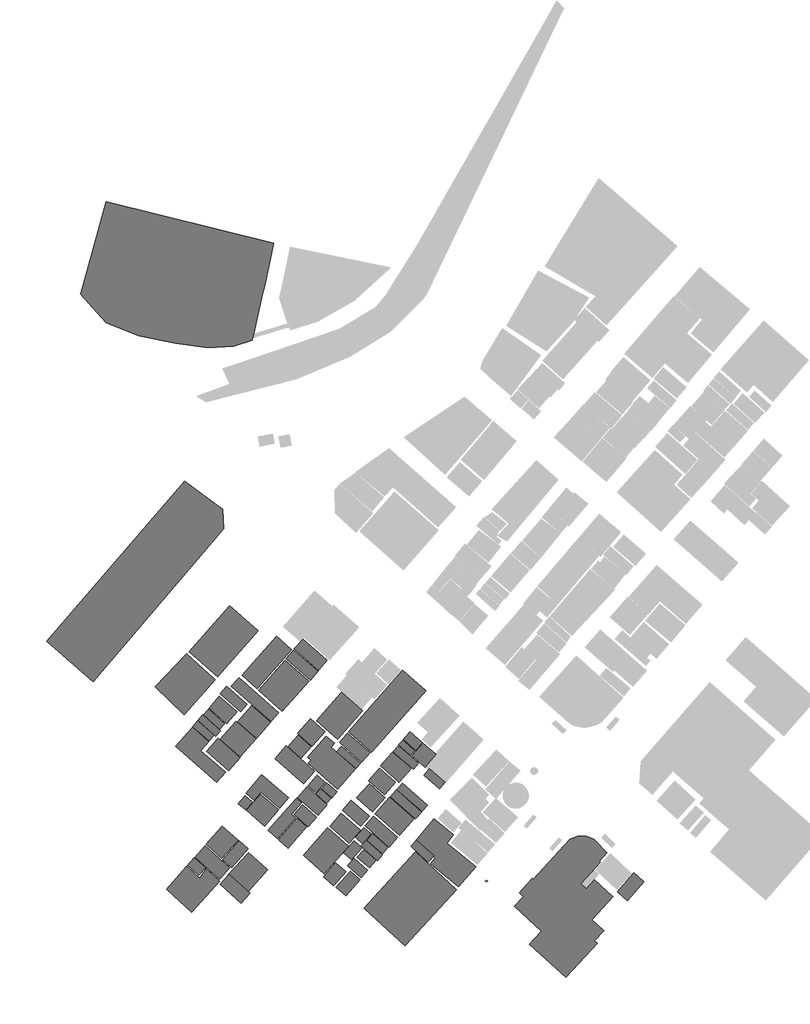
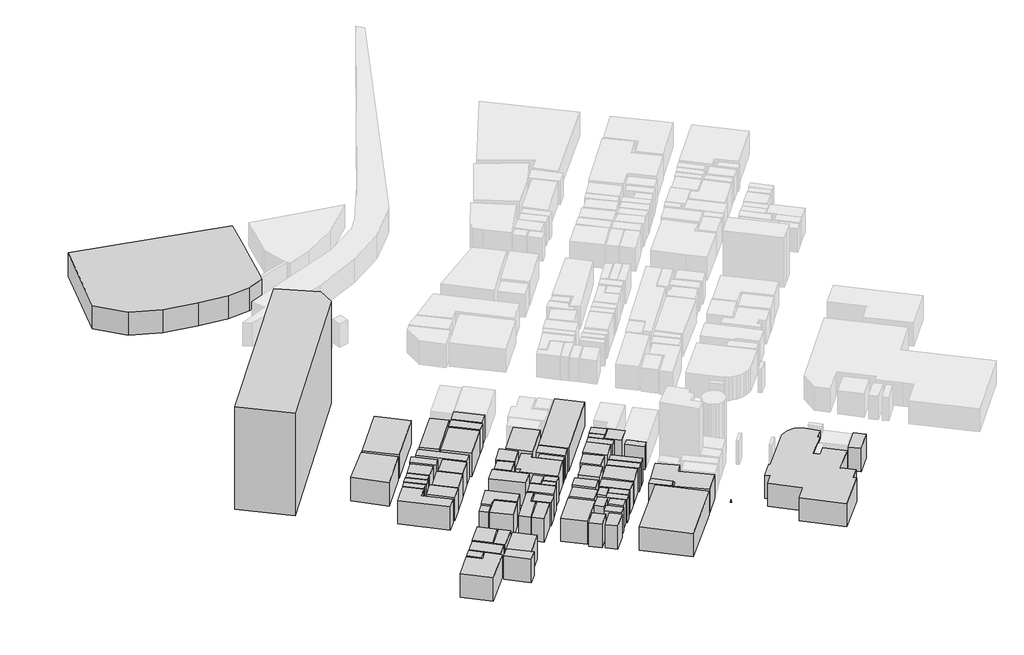
# One storey, part 1 of 3: 72 proxies.
"""IFC4 building model written with IfcOpenShell, lengths in millimetres."""

import ifcopenshell
import ifcopenshell.guid

model = None  # the IFC model being written
_history = None  # IfcOwnerHistory: only IFC2X3 demands one
_inside = {}  # id of a spatial element -> (the spatial element, [elements in it])
_under = {}  # id of a project, library or spatial element -> (it, [spatial elements below it])
_declared = {}  # id of a project -> (the project, [libraries it declares])
_typed = {}  # id of a type object -> (the type object, [elements of that type])
_made_of = {}  # id of a material, layer set ... -> (it, [elements and type objects made of it])


def new_model(schema):
    """Start an empty IFC model of exactly this schema.

    Asked for "IFC4X3", IfcOpenShell would pick the latest addendum, in which some entities
    have other attributes; the version numbers below select the first issue.
    IFC2X3 requires an IfcOwnerHistory on every rooted entity: one is made here for all.
    """
    global model, _history
    if schema == "IFC4X3":
        model = ifcopenshell.file(schema_version=(4, 3, 0, 0))
    else:
        model = ifcopenshell.file(schema=schema)
    _inside.clear()
    _under.clear()
    _declared.clear()
    _typed.clear()
    _made_of.clear()
    _history = None
    if model.schema == "IFC2X3":
        org = make("IfcOrganization", Name="unknown")
        user = make(
            "IfcPersonAndOrganization",
            ThePerson=make("IfcPerson", FamilyName="unknown"),
            TheOrganization=org,
        )
        app = make(
            "IfcApplication",
            ApplicationDeveloper=org,
            Version="unknown",
            ApplicationFullName="unknown",
            ApplicationIdentifier="unknown",
        )
        _history = make(
            "IfcOwnerHistory",
            OwningUser=user,
            OwningApplication=app,
            ChangeAction="ADDED",
            CreationDate=0,
        )
    return model


def make(cls, **values):
    """One entity of the class cls with the attributes given. An attribute that is None is left unset."""
    return model.create_entity(
        cls, **{name: value for name, value in values.items() if value is not None}
    )


def rooted(cls, **values):
    """An entity with a GlobalId (a new one), such as an element, a storey or a relation."""
    return make(cls, GlobalId=ifcopenshell.guid.new(), OwnerHistory=_history, **values)


def si_unit(unit_type, name, prefix=None):
    """IfcSIUnit, for example si_unit("LENGTHUNIT", "METRE", prefix="MILLI")."""
    return make("IfcSIUnit", UnitType=unit_type, Prefix=prefix, Name=name)


def assignment(units):
    """IfcUnitAssignment: the units of a project."""
    return None if units is None else make("IfcUnitAssignment", Units=units)


def point(xyz):
    """IfcCartesianPoint."""
    return None if xyz is None else make("IfcCartesianPoint", Coordinates=xyz)


def direction(xyz):
    """IfcDirection."""
    return None if xyz is None else make("IfcDirection", DirectionRatios=xyz)


def frame(location, z_axis=None, x_axis=None):
    """IfcAxis2Placement3D, a coordinate frame: its origin and axes. An axis left out is left unset."""
    return make(
        "IfcAxis2Placement3D",
        Location=point(location),
        Axis=direction(z_axis),
        RefDirection=direction(x_axis),
    )


def origin():
    """The frame at (0, 0, 0) with its axes left unset."""
    return frame((0.0, 0.0, 0.0))


def origin_with_axes():
    """The frame at (0, 0, 0) with the z axis (0, 0, 1) and the x axis (1, 0, 0) written out."""
    return frame((0.0, 0.0, 0.0), z_axis=(0.0, 0.0, 1.0), x_axis=(1.0, 0.0, 0.0))


def place(relative_to, where):
    """IfcLocalPlacement: puts the frame where relative to a parent placement (None: the world)."""
    return make(
        "IfcLocalPlacement", PlacementRelTo=relative_to, RelativePlacement=where
    )


def context(
    kind, dimensions, precision=None, world=None, true_north=None, identifier=None
):
    """IfcGeometricRepresentationContext, for example the 3D "Model" context."""
    return make(
        "IfcGeometricRepresentationContext",
        ContextIdentifier=identifier,
        ContextType=kind,
        CoordinateSpaceDimension=dimensions,
        Precision=precision,
        WorldCoordinateSystem=world,
        TrueNorth=true_north,
    )


def project(units=None, contexts=None):
    """IfcProject with its units and contexts."""
    return rooted(
        "IfcProject",
        Name="project",
        RepresentationContexts=contexts,
        UnitsInContext=assignment(units),
    )


def spatial(cls, under=None, at=None, **own):
    """A site, building, storey or space (cls), placed at a placement, below another one or the project."""
    s = rooted(cls, ObjectPlacement=at, **own)
    if under is not None:
        _under.setdefault(under.id(), (under, []))[1].append(s)
    return s


def polyline(points):
    """IfcPolyline through the points."""
    return make("IfcPolyline", Points=[point(p) for p in points])


def point_list(points):
    """IfcCartesianPointList2D or 3D."""
    cls = (
        "IfcCartesianPointList2D" if len(points[0]) == 2 else "IfcCartesianPointList3D"
    )
    return make(cls, CoordList=points)


def outline(outer, holes=None, kind="AREA"):
    """IfcArbitraryClosedProfileDef: a profile drawn as a closed curve; with holes, ...WithVoids."""
    if holes is None:
        return make("IfcArbitraryClosedProfileDef", ProfileType=kind, OuterCurve=outer)
    return make(
        "IfcArbitraryProfileDefWithVoids",
        ProfileType=kind,
        OuterCurve=outer,
        InnerCurves=holes,
    )


def extrude(swept, where, along, depth):
    """IfcExtrudedAreaSolid: the profile swept, set in the frame where, extruded along a direction by depth."""
    return make(
        "IfcExtrudedAreaSolid",
        SweptArea=swept,
        Position=where,
        ExtrudedDirection=direction(along),
        Depth=depth,
    )


def triangles(points, corners, closed=None, point_numbers=None):
    """IfcTriangulatedFaceSet: each triangle names its three corners, points numbered from 1."""
    return make(
        "IfcTriangulatedFaceSet",
        Coordinates=point_list(points),
        Closed=closed,
        CoordIndex=corners,
        PnIndex=point_numbers,
    )


def shape(context_of_items, identifier, shape_type, items):
    """IfcShapeRepresentation: the items that make up one representation, for example the "Body"."""
    return make(
        "IfcShapeRepresentation",
        ContextOfItems=context_of_items,
        RepresentationIdentifier=identifier,
        RepresentationType=shape_type,
        Items=items,
    )


def source(mapping_origin, context_of_items, identifier, shape_type, items):
    """IfcRepresentationMap: a shape defined once, which mapped items show again and again."""
    return make(
        "IfcRepresentationMap",
        MappingOrigin=mapping_origin,
        MappedRepresentation=shape(context_of_items, identifier, shape_type, items),
    )


def transform(
    local_origin,
    x_axis=None,
    y_axis=None,
    z_axis=None,
    scale=None,
    scale2=None,
    scale3=None,
    uniform=True,
):
    """IfcCartesianTransformationOperator3D, or its non-uniform kind. x_axis, y_axis, z_axis: its Axis1, 2, 3."""
    if uniform:
        return make(
            "IfcCartesianTransformationOperator3D",
            Axis1=direction(x_axis),
            Axis2=direction(y_axis),
            LocalOrigin=point(local_origin),
            Scale=scale,
            Axis3=direction(z_axis),
        )
    return make(
        "IfcCartesianTransformationOperator3DnonUniform",
        Axis1=direction(x_axis),
        Axis2=direction(y_axis),
        LocalOrigin=point(local_origin),
        Scale=scale,
        Axis3=direction(z_axis),
        Scale2=scale2,
        Scale3=scale3,
    )


def mapped(mapping_source, mapping_target):
    """IfcMappedItem: shows the shape of a source again, moved by a transform."""
    return make(
        "IfcMappedItem", MappingSource=mapping_source, MappingTarget=mapping_target
    )


def made_of(thing, what):
    """Note that an element or type object is made of a material, layer set ...; save() writes the relation."""
    if what is not None:
        _made_of.setdefault(what.id(), (what, []))[1].append(thing)
    return thing


def element(
    cls,
    number,
    at=None,
    inside=None,
    cuts=None,
    type_object=None,
    material=None,
    context=None,
    identifier="Body",
    shape_type=None,
    held_by="IfcProductDefinitionShape",
    body=None,
    shapes=None,
    **own,
):
    """One element of the class cls, such as IfcWall. Its Tag is "e" and its number.

    at: its placement. inside: the storey or other place that contains it. cuts: it is an
    opening in that element (IfcRelVoidsElement). A single representation is given by context,
    identifier, shape_type and body (its items); several are given by shapes. held_by: the class
    of the entity that holds the representations. save() writes the other relations.
    """
    e = rooted(cls, Tag="e%d" % number, ObjectPlacement=at, **own)
    if body is not None:
        shapes = [shape(context, identifier, shape_type, body)]
    if shapes is not None:
        e.Representation = make(held_by, Representations=shapes)
    if inside is not None:
        _inside.setdefault(inside.id(), (inside, []))[1].append(e)
    if cuts is not None:
        rooted(
            "IfcRelVoidsElement", RelatingBuildingElement=cuts, RelatedOpeningElement=e
        )
    if type_object is not None:
        _typed.setdefault(type_object.id(), (type_object, []))[1].append(e)
    return made_of(e, material)


def aggregate(whole, parts):
    """IfcRelAggregates: a whole, such as a stair, and the parts it consists of."""
    return rooted("IfcRelAggregates", RelatingObject=whole, RelatedObjects=parts)


def save(model, path):
    """Write the relations noted so far, then the file.

    IfcRelAggregates (storeys below a building ...), IfcRelContainedInSpatialStructure (elements
    in a storey), IfcRelDefinesByType, IfcRelAssociatesMaterial and IfcRelDeclares: one each for
    every whole, place, type object, material and project.
    """
    for whole, parts in _under.values():
        aggregate(whole, parts)
    for where, things in _inside.values():
        rooted(
            "IfcRelContainedInSpatialStructure",
            RelatedElements=things,
            RelatingStructure=where,
        )
    for kind, things in _typed.values():
        rooted("IfcRelDefinesByType", RelatedObjects=things, RelatingType=kind)
    for what, things in _made_of.values():
        rooted("IfcRelAssociatesMaterial", RelatedObjects=things, RelatingMaterial=what)
    for by, libraries in _declared.values():
        rooted("IfcRelDeclares", RelatingContext=by, RelatedDefinitions=libraries)
    model.write(path)


def m_rpc_female_e5f04239(model_context):
    return source(origin(), model_context, "Body", "Tessellation", [
        triangles([(-437.3057565, 0.0, 2.93e-05), (-425.7448342, -100.2015691, 2.93e-05), (-392.8194094, -192.2206799, 2.93e-05), (-341.1658762, -273.4208834, 2.93e-05), (-273.4209015, -341.1659489, 2.93e-05), (-192.2206254, -392.819373, 2.93e-05), (-100.2015237, -425.7447979, 2.93e-05), (1.91e-05, -437.3057565, 2.93e-05), (100.2015782, -425.7448342, 2.93e-05), (192.220698, -392.8194094, 2.93e-05), (273.4209015, -341.1658762, 2.93e-05), (341.1660215, -273.4209015, 2.93e-05), (392.819373, -192.2206072, 2.93e-05), (425.7447979, -100.2014965, 2.93e-05), (437.3057565, 3.36e-05, 2.93e-05), (-5.73e-05, 437.3057928, 2.93e-05), (-5.5814555, 72.246871, 69.496344), (-5.5814561, 67.031142, 46.0256608), (-5.5814583, 124.4039254, 19.9471336), (-5.5814583, 129.6196318, 25.1628196), (-5.5814566, 107.6002273, 62.2269385), (-5.5814561, 95.7175496, 74.7120321), (-5.5814561, -28.6037069, 4.4e-06), (-5.5814555, -39.8908654, 35.5942482), (-5.5814555, -42.4985551, 37.2668205), (-5.5814544, -45.6385706, 39.1828009), (-5.5814544, -48.9915363, 41.1595652), (-5.5814544, -52.2381223, 43.0148345), (-5.5814544, -55.0589122, 44.56573), (-5.5814544, -57.1346076, 45.6302408), (-5.5814544, -58.1458059, 46.0256654), (-5.5814555, -58.1458876, 5.3e-06), (-5.5814555, -108.9534241, 6.8e-06), (-5.5814544, -116.5758149, 29.8220214), (-5.5814504, -109.3236867, 163.616957), (-5.5814413, -45.457159, 488.7457126), (-5.5814407, -47.714434, 510.223653), (-5.5814407, -52.9301222, 512.8314517), (-5.5814407, -176.6935208, 461.1352976), (-5.5814373, -431.0100652, 441.4516517), (-5.5814373, -446.7160832, 445.0273055), (-5.5814368, -456.1585665, 455.8251566), (-5.58143, -511.6809405, 636.0529638), (-5.581426, -514.5203021, 776.2247131), (-5.5814186, -566.7671494, 1012.4528812), (-5.5814158, -561.4616592, 1112.6378271), (-5.5814129, -522.3438071, 1198.6970364), (-5.5814129, -544.7658397, 1204.5966036), (-5.5814118, -561.2097487, 1214.9815075), (-5.5814118, -573.9143148, 1236.2570984), (-5.5814101, -577.4586843, 1272.8740494), (-5.5814084, -566.4219306, 1329.2825249), (-5.5814067, -535.3830912, 1409.9332706), (-5.5814067, -516.7872059, 1433.7636475), (-5.5814055, -472.5754423, 1474.3204742), (-5.5814055, -445.9832065, 1486.7813416), (-5.5814067, -415.7490417, 1491.1880493), (-5.5814067, -381.3846422, 1485.4068615), (-5.5814084, -308.1102631, 1450.1703495), (-5.5814101, -271.6907746, 1426.3735462), (-5.5814107, -259.9822778, 1410.5514015), (-5.5814118, -256.5008769, 1391.3528641), (-5.5814118, -264.1662884, 1368.2074745), (-5.5814118, -270.5525991, 1361.5164585), (-5.5814118, -307.4893707, 1345.9730759), (-5.5814118, -313.6895373, 1341.0963387), (-5.5814118, -316.3233519, 1334.3053288), (-5.5814129, -314.5104538, 1321.5896805), (-5.5814141, -303.2841405, 1289.971843), (-5.5814141, -303.9328654, 1281.3184467), (-5.5814146, -344.8551496, 1227.4567635), (-5.5814158, -350.2254976, 1216.9519541), (-5.5814158, -354.0100413, 1213.137216), (-5.5814158, -360.9104559, 1211.8311184), (-5.5814146, -397.1668911, 1216.9519541), (-5.5814158, -412.8139375, 1162.1870556), (-5.581422, -300.7217424, 1007.464959), (-5.581426, -262.9222146, 903.7019611), (-5.5814277, -261.5584715, 849.2446747), (-5.58143, -151.2454102, 828.1022152), (-5.58143, -131.1657765, 828.3817766), (-5.5814288, -146.9133073, 873.4847649), (-5.5814288, -146.8129046, 875.3230974), (-5.5814288, -136.5283852, 880.5989382), (-5.581426, 66.2908528, 1062.7618744), (-5.581426, 72.9541861, 1068.1172161), (-5.5814266, 85.3175848, 1063.7719145), (-5.5814322, 186.9119923, 916.7356859), (-5.5814328, 189.6002729, 904.0095005), (-5.5814339, 74.8547106, 802.3032812), (-5.5814345, 53.5231683, 768.5290346), (-5.5814345, 40.9526102, 757.9697954), (-5.5814345, 7.0502408, 750.1462177), (-5.5814362, -30.7395663, 681.3427139), (-5.5814362, -32.0672787, 677.1262562), (-5.5814368, -2.7970168, 673.1418337), (-5.5814379, 74.8547106, 666.6947708), (-5.5814566, 223.5023279, 113.8298615), (-5.5814572, 192.3027606, 86.4272282), (-5.5814572, 189.6002729, 82.5355962), (-5.5814595, 257.4045281, 53.849234), (-5.5814595, 261.0572667, 50.6335418), (-5.5814595, 266.9932234, 41.9573409), (-5.58146, 270.4022813, 33.1798288), (-5.58146, 270.8965462, 29.8373185), (-5.58146, 270.443685, 27.7706614), (-5.58146, 262.21192, 24.6723971), (-5.5814583, 148.3989361, 17.7234776), (-5.5814583, 129.6196318, 12.1235594), (-5.5814583, 119.2279423, 0.0), (-103.2161017, -158.8625416, 3.138314), (-93.5649194, -158.8625416, 19.242982), (-88.6211895, -158.8625416, 24.4594286), (-82.9717796, -158.8625416, 28.4095146), (-76.7113605, -158.8625416, 30.3784918), (-108.0056168, -158.8625779, 484.1449396), (-166.5178156, -158.8625779, 527.9969504), (-183.6322324, -158.8625779, 549.73316), (-196.1559229, -158.8625779, 575.232294), (-202.0512208, -158.8625779, 604.6166196), (-199.2805142, -158.8625779, 638.0082951), (-180.7337175, -158.8625779, 688.9249546), (-179.5104455, -158.8625779, 700.1737593), (-181.025542, -158.8625779, 711.0281839), (-186.0298695, -158.8625779, 724.8027792), (-192.7431225, -158.8625779, 739.7135696), (-208.5562016, -158.8625779, 771.7149593), (-227.9668809, -158.8625779, 820.5580536), (-215.5926726, -158.8626143, 1139.7189503), (-204.4961842, -158.8626143, 1164.7947453), (-195.70417, -158.8626143, 1170.2244284), (-178.399812, -158.8626143, 1176.5899555), (-156.0960135, -158.8626143, 1183.4364126), (-132.3055416, -158.8626143, 1190.3077229), (-110.5413086, -158.8626143, 1196.7492628), (-94.3160908, -158.8626143, 1202.3054644), (-87.1427823, -158.8626143, 1206.520396), (-121.0448735, -158.8626143, 1339.5209988), (-105.9598205, -158.8626324, 1402.4766037), (-72.2006347, -158.8626324, 1459.392897), (-51.1398926, -158.8626324, 1480.6086079), (-28.7965572, -158.8626324, 1494.3413452), (-6.2993123, -158.8626324, 1498.5999516), (28.3785935, -158.8626324, 1491.3003971), (62.9443729, -158.8626324, 1473.3395748), (92.2084342, -158.8626324, 1445.5309525), (103.2305721, -158.8626324, 1428.1879704), (112.1216355, -158.8626324, 1400.9896305), (114.2135136, -158.8626143, 1329.2264236), (96.1614451, -158.8626143, 1258.9092041), (79.8725593, -158.8626143, 1233.5183121), (58.89705, -158.8626143, 1219.5597164), (58.89705, -158.8626143, 1209.128231), (105.4402574, -158.8626143, 1177.1569994), (186.6818646, -158.8626143, 1146.5396822), (190.9101676, -158.8626143, 1130.2527403), (197.4604945, -158.8625961, 874.5614433), (217.1152177, -158.8625961, 870.6124111), (219.4354431, -158.8625961, 869.5266489), (221.3548754, -158.8625961, 866.986179), (227.9668991, -158.8625779, 839.7665468), (217.9761209, -158.8625779, 726.675412), (216.778683, -158.8625779, 725.536964), (198.418848, -158.8625779, 721.3532078), (197.1132955, -158.8625779, 721.4596693), (188.2934486, -158.8625779, 736.0850121), (176.2504519, -158.8625779, 750.1460724), (172.5434834, -158.8625779, 744.3784012), (169.4576071, -158.8625779, 737.6237263), (166.7654749, -158.8625779, 730.2867468), (164.2397206, -158.8625779, 722.7717985), (161.6530689, -158.8625779, 715.4834352), (158.7781536, -158.8625779, 708.8262835), (155.3876265, -158.8625779, 703.2046789), (164.598783, -158.8625779, 582.3864721), (159.7288041, -158.8625779, 557.993666), (150.1719383, -158.8625779, 536.3020758), (143.4521541, -158.8625779, 528.6086137), (105.433708, -158.8625779, 509.5447337), (96.8765541, -158.8625779, 503.2554737), (90.1912608, -158.8625779, 494.5763523), (88.7455914, -158.8625416, 49.4103652), (105.4366057, -158.8625416, 7.4e-05), (-104.3910027, -158.8625416, 7.4e-05)], [[15, 16, 1], [14, 15, 1], [14, 1, 2], [13, 14, 2], [13, 2, 3], [13, 3, 4], [12, 13, 4], [11, 12, 4], [11, 4, 5], [11, 5, 6], [11, 6, 7], [11, 7, 8], [11, 8, 9], [11, 9, 10], [23, 17, 18], [110, 23, 18], [110, 18, 19], [109, 110, 19], [17, 23, 24], [31, 32, 33], [31, 33, 34], [109, 19, 20], [108, 109, 20], [88, 89, 90], [82, 83, 84], [85, 86, 87], [105, 106, 107], [104, 105, 107], [103, 104, 107], [102, 103, 107], [101, 102, 107], [100, 101, 107], [100, 107, 108], [100, 108, 20], [100, 20, 21], [100, 21, 22], [87, 88, 90], [85, 87, 90], [84, 85, 90], [84, 90, 91], [84, 91, 92], [84, 92, 93], [82, 84, 93], [81, 82, 93], [81, 93, 94], [80, 81, 94], [80, 94, 95], [99, 100, 22], [17, 24, 25], [17, 25, 26], [31, 34, 35], [30, 31, 35], [17, 26, 27], [17, 27, 28], [17, 28, 29], [29, 30, 35], [17, 29, 35], [22, 17, 35], [99, 22, 35], [98, 99, 35], [97, 98, 35], [97, 35, 36], [97, 36, 37], [96, 97, 37], [96, 37, 38], [95, 96, 38], [80, 95, 38], [80, 38, 39], [79, 80, 39], [79, 39, 40], [79, 40, 41], [79, 41, 42], [79, 42, 43], [79, 43, 44], [78, 79, 44], [77, 78, 44], [77, 44, 45], [77, 45, 46], [76, 77, 46], [76, 46, 47], [75, 76, 47], [72, 73, 74], [71, 72, 74], [61, 62, 63], [60, 61, 63], [60, 63, 64], [59, 60, 64], [59, 64, 65], [59, 65, 66], [58, 59, 66], [57, 58, 66], [56, 57, 66], [55, 56, 66], [54, 55, 66], [54, 66, 67], [53, 54, 67], [52, 53, 67], [52, 67, 68], [51, 52, 68], [50, 51, 68], [49, 50, 68], [48, 49, 68], [47, 48, 68], [75, 47, 68], [74, 75, 68], [71, 74, 68], [70, 71, 68], [69, 70, 68], [183, 184, 111], [183, 111, 112], [183, 112, 113], [183, 113, 114], [183, 114, 115], [182, 183, 115], [181, 182, 115], [181, 115, 116], [154, 155, 156], [164, 165, 166], [180, 181, 116], [163, 164, 166], [162, 163, 166], [162, 166, 167], [161, 162, 167], [160, 161, 167], [159, 160, 167], [158, 159, 167], [157, 158, 167], [180, 116, 117], [180, 117, 118], [180, 118, 119], [180, 119, 120], [180, 120, 121], [180, 121, 122], [179, 180, 122], [179, 122, 123], [178, 179, 123], [177, 178, 123], [176, 177, 123], [175, 176, 123], [174, 175, 123], [174, 123, 124], [174, 124, 125], [173, 174, 125], [172, 173, 125], [171, 172, 125], [170, 171, 125], [169, 170, 125], [169, 125, 126], [168, 169, 126], [168, 126, 127], [167, 168, 127], [157, 167, 127], [157, 127, 128], [156, 157, 128], [154, 156, 128], [153, 154, 128], [153, 128, 129], [153, 129, 130], [153, 130, 131], [153, 131, 132], [153, 132, 133], [153, 133, 134], [153, 134, 135], [153, 135, 136], [153, 136, 137], [152, 153, 137], [151, 152, 137], [150, 151, 137], [149, 150, 137], [149, 137, 138], [149, 138, 139], [148, 149, 139], [147, 148, 139], [146, 147, 139], [146, 139, 140], [145, 146, 140], [145, 140, 141], [144, 145, 141], [144, 141, 142], [144, 142, 143]], closed=False),
    ])


model = new_model("IFC4")

# Units and contexts
model_context = context("Model", 3, world=origin())
ifc_project = project(units=[si_unit("LENGTHUNIT", "METRE", prefix="MILLI")], contexts=[model_context])

# Site, building, storey
site = spatial("IfcSite", under=ifc_project)
building = spatial("IfcBuilding", under=site)
storey = spatial("IfcBuildingStorey", under=building, Name="レベル 0", Elevation=0.0)

# Proxies
placement = place(None, origin())
element("IfcBuildingElementProxy", 1, Name="Mass", at=placement, inside=storey, context=model_context, shape_type="SweptSolid", body=[
    extrude(outline(polyline([(-81027.0217269, 125127.6509537), (-8762.1194073, 208768.4747751), (11065.563168, 193957.3105467), (11679.8148372, 183871.9306999), (-56475.0211631, 103911.6589493), (-81027.0217269, 125127.6509537)])), origin_with_axes(), (0.0, 0.0, 1.0), 66000.0),
])
element("IfcBuildingElementProxy", 2, Name="Mass", at=placement, inside=storey, context=model_context, shape_type="SweptSolid", body=[
    extrude(outline(polyline([(60169.5642931, 83373.9559982), (73321.7765149, 98307.4346465), (84306.0416675, 88633.4760284), (71144.7963334, 73699.9973801), (60169.5642931, 83373.9559982)])), origin_with_axes(), (0.0, 0.0, 1.0), 15000.0),
])
element("IfcBuildingElementProxy", 3, Name="Mass", at=placement, inside=storey, context=model_context, shape_type="SweptSolid", body=[
    extrude(outline(polyline([(2438.9404523, 18836.4205741), (10893.9340249, 28276.8698459), (19105.0335488, 20926.8851949), (10650.0399787, 11475.3164303), (2438.9404523, 18836.4205741)])), origin_with_axes(), (0.0, 0.0, 1.0), 15000.0),
])
element("IfcBuildingElementProxy", 4, Name="Mass", at=placement, inside=storey, context=model_context, shape_type="SweptSolid", body=[
    extrude(outline(polyline([(85191.2867223, 27565.2223158), (88867.7636278, 24318.3304577), (84405.4059075, 19258.9612947), (80728.929002, 22494.7336608), (85191.2867223, 27565.2223158)])), origin_with_axes(), (0.0, 0.0, 1.0), 15000.0),
])
element("IfcBuildingElementProxy", 5, Name="Mass", at=placement, inside=storey, context=model_context, shape_type="SweptSolid", body=[
    extrude(outline(polyline([(76944.0547443, 77691.8952467), (105371.2606935, 109960.6629591), (117538.8636232, 99230.3525382), (89120.6907837, 66972.7043185), (76944.0547443, 77691.8952467)])), origin_with_axes(), (0.0, 0.0, 1.0), 15000.0),
])
element("IfcBuildingElementProxy", 6, Name="Mass", at=placement, inside=storey, context=model_context, shape_type="SweptSolid", body=[
    extrude(outline(polyline([(105479.6580482, 73344.1736146), (111622.1747453, 67928.9806877), (109400.0289974, 65415.9753454), (103248.4791881, 70820.0487803), (105479.6580482, 73344.1736146)])), origin_with_axes(), (0.0, 0.0, 1.0), 15000.0),
])
element("IfcBuildingElementProxy", 7, Name="Mass", at=placement, inside=storey, context=model_context, shape_type="SweptSolid", body=[
    extrude(outline(polyline([(65986.8889311, 27531.8638374), (76907.9222927, 17913.5026824), (64279.6306124, 3580.4766379), (53358.5972507, 13198.8377929), (65986.8889311, 27531.8638374)])), origin_with_axes(), (0.0, 0.0, 1.0), 15000.0),
])
element("IfcBuildingElementProxy", 8, Name="Mass", at=placement, inside=storey, context=model_context, shape_type="SweptSolid", body=[
    extrude(outline(polyline([(81496.7435898, 12142.4859901), (85010.6244644, 16134.3838566), (91424.1345471, 10485.6815827), (87910.2536699, 6493.7837161), (81496.7435898, 12142.4859901)])), origin_with_axes(), (0.0, 0.0, 1.0), 15000.0),
])
element("IfcBuildingElementProxy", 9, Name="Mass", at=placement, inside=storey, context=model_context, shape_type="SweptSolid", body=[
    extrude(outline(polyline([(-1878.8874617, 83362.8365054), (6657.4041263, 75834.9399721), (4082.96698, 72910.5134012), (-4453.3246055, 80427.2904425), (-1878.8874617, 83362.8365054)])), origin_with_axes(), (0.0, 0.0, 1.0), 15000.0),
])
element("IfcBuildingElementProxy", 10, Name="Mass", at=placement, inside=storey, context=model_context, shape_type="SweptSolid", body=[
    extrude(outline(polyline([(3676.4769055, 89478.5574712), (12266.9671671, 81906.1829667), (9674.4637962, 78970.636903), (1083.9735346, 86543.0114075), (3676.4769055, 89478.5574712)])), origin_with_axes(), (0.0, 0.0, 1.0), 15000.0),
])
element("IfcBuildingElementProxy", 11, Name="Mass", at=placement, inside=storey, context=model_context, shape_type="SweptSolid", body=[
    extrude(outline(polyline([(13179.3115586, 101509.8485342), (23883.550216, 92080.5187543), (20514.1991451, 88266.5327709), (9818.9936026, 97695.8625499), (13179.3115586, 101509.8485342)])), origin_with_axes(), (0.0, 0.0, 1.0), 15000.0),
])
element("IfcBuildingElementProxy", 12, Name="Mass", at=placement, inside=storey, context=model_context, shape_type="SweptSolid", body=[
    extrude(outline(polyline([(62762.0676639, 48025.088818), (65499.1008385, 51127.4272713), (70982.2003026, 46290.4479627), (68245.167128, 43188.1095094), (62762.0676639, 48025.088818)])), origin_with_axes(), (0.0, 0.0, 1.0), 15000.0),
])
element("IfcBuildingElementProxy", 13, Name="Mass", at=placement, inside=storey, context=model_context, shape_type="SweptSolid", body=[
    extrude(outline(polyline([(18174.6229327, 83262.7610719), (28625.9344316, 74066.9406383), (20342.570002, 64670.9693369), (9900.291618, 73877.9092632), (18174.6229327, 83262.7610719)])), origin_with_axes(), (0.0, 0.0, 1.0), 15000.0),
])
element("IfcBuildingElementProxy", 14, Name="Mass", at=placement, inside=storey, context=model_context, shape_type="SweptSolid", body=[
    extrude(outline(polyline([(109689.0886075, 17835.6662344), (112670.0158283, 21093.6775845), (121685.0623915, 12843.0140274), (118695.1020584, 9585.0026774), (109689.0886075, 17835.6662344)])), origin_with_axes(), (0.0, 0.0, 1.0), 15000.0),
])
element("IfcBuildingElementProxy", 15, Name="Mass", at=placement, inside=storey, context=model_context, shape_type="SweptSolid", body=[
    extrude(outline(polyline([(76537.5646672, 7572.3745045), (79961.1144168, 11464.1969375), (87043.0748422, 5226.1615525), (83619.5250952, 1334.3391203), (76537.5646672, 7572.3745045)])), origin_with_axes(), (0.0, 0.0, 1.0), 15000.0),
])
element("IfcBuildingElementProxy", 16, Name="Mass", at=placement, inside=storey, context=model_context, shape_type="SweptSolid", body=[
    extrude(outline(polyline([(23630.6230575, 36694.3257933), (31064.8748838, 45134.0207255), (40432.212848, 36883.3571684), (32997.9610217, 28443.6622362), (23630.6230575, 36694.3257933)])), origin_with_axes(), (0.0, 0.0, 1.0), 15000.0),
])
element("IfcBuildingElementProxy", 17, Name="Mass", at=placement, inside=storey, context=model_context, shape_type="SweptSolid", body=[
    extrude(outline(polyline([(78271.9223252, 41931.6068378), (87919.2867847, 33436.3144425), (83393.697276, 28299.1088315), (73737.2997043, 36794.4012269), (78271.9223252, 41931.6068378)])), origin_with_axes(), (0.0, 0.0, 1.0), 15000.0),
])
element("IfcBuildingElementProxy", 18, Name="Mass", at=placement, inside=storey, context=model_context, shape_type="SweptSolid", body=[
    extrude(outline(polyline([(93673.3796317, 59833.9900274), (100095.9228241, 67128.3772152), (109851.6846383, 58533.0093863), (103429.1414434, 51238.6221977), (93673.3796317, 59833.9900274)])), origin_with_axes(), (0.0, 0.0, 1.0), 15000.0),
])
element("IfcBuildingElementProxy", 19, Name="Mass", at=placement, inside=storey, context=model_context, shape_type="SweptSolid", body=[
    extrude(outline(polyline([(116572.320553, 55063.7276747), (119408.7179701, 58288.3805472), (127366.890338, 51271.9806761), (124521.4598087, 48047.3278036), (116572.320553, 55063.7276747)])), origin_with_axes(), (0.0, 0.0, 1.0), 15000.0),
])
element("IfcBuildingElementProxy", 20, Name="Mass", at=placement, inside=storey, context=model_context, shape_type="SweptSolid", body=[
    extrude(outline(polyline([(85516.4787814, 28499.2596994), (90069.1676269, 33658.7042952), (102688.4261949, 22539.2116311), (98135.7373495, 17379.7670346), (85516.4787814, 28499.2596994)])), origin_with_axes(), (0.0, 0.0, 1.0), 15000.0),
])
element("IfcBuildingElementProxy", 21, Name="Mass", at=placement, inside=storey, context=model_context, shape_type="SweptSolid", body=[
    extrude(outline(polyline([(40350.9148326, 21360.5454084), (50052.4779682, 32379.9626388), (55065.8555668, 27954.4045588), (45364.2924312, 16934.9873283), (40350.9148326, 21360.5454084)])), origin_with_axes(), (0.0, 0.0, 1.0), 15000.0),
])
element("IfcBuildingElementProxy", 22, Name="Mass", at=placement, inside=storey, context=model_context, shape_type="SweptSolid", body=[
    extrude(outline(polyline([(45490.7560105, 69930.489367), (50720.928316, 75868.2984497), (57504.7960191, 69897.1308886), (52265.5906013, 63959.321806), (45490.7560105, 69930.489367)])), origin_with_axes(), (0.0, 0.0, 1.0), 15000.0),
])
element("IfcBuildingElementProxy", 23, Name="Mass", at=placement, inside=storey, context=model_context, shape_type="SweptSolid", body=[
    extrude(outline(polyline([(29818.3053184, 99430.5034061), (43693.1665642, 115175.7050189), (56222.0940046, 104134.0488028), (42347.2327588, 88388.84719), (29818.3053184, 99430.5034061)])), origin_with_axes(), (0.0, 0.0, 1.0), 15000.0),
])
element("IfcBuildingElementProxy", 24, Name="Mass", at=placement, inside=storey, context=model_context, shape_type="SweptSolid", body=[
    extrude(outline(polyline([(55743.3390269, 49526.2203279), (60585.0874824, 55019.2497043), (64785.4849294, 51316.4586465), (59943.7364739, 45823.4292708), (55743.3390269, 49526.2203279)])), origin_with_axes(), (0.0, 0.0, 1.0), 15000.0),
])
element("IfcBuildingElementProxy", 25, Name="Mass", at=placement, inside=storey, context=model_context, shape_type="SweptSolid", body=[
    extrude(outline(polyline([(76546.5977821, 77024.7256869), (88226.4126193, 66728.0754794), (83926.6509298, 61846.6182003), (72237.8029803, 72143.268407), (76546.5977821, 77024.7256869)])), origin_with_axes(), (0.0, 0.0, 1.0), 15000.0),
])
element("IfcBuildingElementProxy", 26, Name="Mass", at=placement, inside=storey, context=model_context, shape_type="SweptSolid", body=[
    extrude(outline(polyline([(19637.9872051, 105991.0040781), (40396.0803965, 87699.4386447), (36439.5769931, 83207.1636087), (15681.4838018, 101498.7290414), (19637.9872051, 105991.0040781)])), origin_with_axes(), (0.0, 0.0, 1.0), 15000.0),
])
element("IfcBuildingElementProxy", 27, Name="Mass", at=placement, inside=storey, context=model_context, shape_type="SweptSolid", body=[
    extrude(outline(polyline([(44334.5175727, 115909.5915346), (48318.1203128, 120424.1055562), (60991.5775569, 109260.134921), (57007.9748169, 104734.5014066), (44334.5175727, 115909.5915346)])), origin_with_axes(), (0.0, 0.0, 1.0), 15000.0),
])
element("IfcBuildingElementProxy", 28, Name="Mass", at=placement, inside=storey, context=model_context, shape_type="SweptSolid", body=[
    extrude(outline(polyline([(98903.5519373, 43821.9205908), (101974.8102858, 47302.3217951), (115099.9231684, 35738.049424), (112028.6648198, 32257.6482197), (98903.5519373, 43821.9205908)])), origin_with_axes(), (0.0, 0.0, 1.0), 15000.0),
])
element("IfcBuildingElementProxy", 29, Name="Mass", at=placement, inside=storey, context=model_context, shape_type="SweptSolid", body=[
    extrude(outline(polyline([(226171.0780354, 3936.3004034), (231446.4159048, -611.5720966), (222837.8594161, -10607.9960018), (217562.5215467, -6060.1235018), (226171.0780354, 3936.3004034)])), origin_with_axes(), (0.0, 0.0, 1.0), 15000.0),
])
element("IfcBuildingElementProxy", 30, Name="Mass", at=placement, inside=storey, context=model_context, shape_type="SweptSolid", body=[
    extrude(outline(polyline([(14118.7552895, 2902.1875854), (24624.2654644, 14566.5353908), (34614.8882101, 5570.8658252), (24100.3449229, -6093.4819802), (14118.7552895, 2902.1875854)])), origin_with_axes(), (0.0, 0.0, 1.0), 15000.0),
])
element("IfcBuildingElementProxy", 31, Name="Mass", at=placement, inside=storey, context=model_context, shape_type="SweptSolid", body=[
    extrude(outline(polyline([(67829.6439386, 69685.8605287), (80647.6309891, 58388.4559815), (71171.8956702, 47635.906575), (55842.7032668, 61134.9706694), (57324.1337637, 62814.0140616), (55499.4449806, 64426.3404978), (65246.17368, 75490.2356994), (69573.0347063, 71676.2497152), (67829.6439386, 69685.8605287)])), origin_with_axes(), (0.0, 0.0, 1.0), 15000.0),
])
element("IfcBuildingElementProxy", 32, Name="Mass", at=placement, inside=storey, context=model_context, shape_type="SweptSolid", body=[
    extrude(outline(polyline([(19773.4838966, 20660.017371), (24488.7687729, 16434.6101581), (15726.6493656, 6649.4566136), (11011.3644894, 10874.8638257), (19773.4838966, 20660.017371)])), origin_with_axes(), (0.0, 0.0, 1.0), 15000.0),
])
element("IfcBuildingElementProxy", 33, Name="Mass", at=placement, inside=storey, context=model_context, shape_type="SweptSolid", body=[
    extrude(outline(polyline([(9773.8280387, -1968.1502017), (14498.1460273, 3269.1308436), (25554.676083, -6682.8150912), (20830.3580919, -11931.2156285), (9773.8280387, -1968.1502017)])), origin_with_axes(), (0.0, 0.0, 1.0), 15000.0),
])
element("IfcBuildingElementProxy", 34, Name="Mass", at=placement, inside=storey, context=model_context, shape_type="SweptSolid", body=[
    extrude(outline(polyline([(-3251.9206065, 12164.7249749), (2005.3510384, 18035.8171024), (14769.1394103, 6616.0981352), (9502.8346531, 733.8865157), (-3251.9206065, 12164.7249749)])), origin_with_axes(), (0.0, 0.0, 1.0), 15000.0),
])
element("IfcBuildingElementProxy", 35, Name="Mass", at=placement, inside=storey, context=model_context, shape_type="SweptSolid", body=[
    extrude(outline(polyline([(74478.0149527, 14410.8624933), (79961.1144168, 20626.6588926), (83989.8827207, 17079.5407331), (78506.7832566, 10863.7443337), (74478.0149527, 14410.8624933)])), origin_with_axes(), (0.0, 0.0, 1.0), 15000.0),
])
element("IfcBuildingElementProxy", 36, Name="Mass", at=placement, inside=storey, context=model_context, shape_type="SweptSolid", body=[
    extrude(outline(polyline([(8689.8545041, 74267.0915063), (20152.8746344, 64092.7557179), (14227.1526442, 57421.0601195), (2773.1656262, 67595.3959079), (8689.8545041, 74267.0915063)])), origin_with_axes(), (0.0, 0.0, 1.0), 15000.0),
])
element("IfcBuildingElementProxy", 37, Name="Mass", at=placement, inside=storey, context=model_context, shape_type="SweptSolid", body=[
    extrude(outline(polyline([(110140.7442484, 65137.9880287), (116048.4000115, 71843.0421055), (122832.2677171, 65871.8745445), (116915.5788392, 59155.7009749), (110140.7442484, 65137.9880287)])), origin_with_axes(), (0.0, 0.0, 1.0), 15000.0),
])
element("IfcBuildingElementProxy", 38, Name="Mass", at=placement, inside=storey, context=model_context, shape_type="SweptSolid", body=[
    extrude(outline(polyline([(73186.2798234, 34993.0434155), (83213.0350207, 26164.1662395), (77251.1805789, 19392.3952067), (67224.4253817, 28232.3918755), (73186.2798234, 34993.0434155)])), origin_with_axes(), (0.0, 0.0, 1.0), 15000.0),
])
element("IfcBuildingElementProxy", 39, Name="Mass", at=placement, inside=storey, context=model_context, shape_type="SweptSolid", body=[
    extrude(outline(polyline([(109165.168066, 77736.3732178), (115614.8105976, 72054.3124663), (112118.9959475, 68084.6535845), (105678.3865281, 73766.7143361), (109165.168066, 77736.3732178)])), origin_with_axes(), (0.0, 0.0, 1.0), 15000.0),
])
element("IfcBuildingElementProxy", 40, Name="Mass", at=placement, inside=storey, context=model_context, shape_type="SweptSolid", body=[
    extrude(outline(polyline([(70530.5446642, -3591.5961307), (77946.7302635, 4825.8598167), (83131.7370052, 255.7483319), (75715.5514034, -8150.5881227), (70530.5446642, -3591.5961307)])), origin_with_axes(), (0.0, 0.0, 1.0), 15000.0),
])
element("IfcBuildingElementProxy", 41, Name="Mass", at=placement, inside=storey, context=model_context, shape_type="SweptSolid", body=[
    extrude(outline(polyline([(59988.9020377, 45211.8571742), (62328.4782501, 47880.5354133), (67947.0744056, 42932.3611775), (65598.465081, 40263.6829384), (59988.9020377, 45211.8571742)])), origin_with_axes(), (0.0, 0.0, 1.0), 15000.0),
])
element("IfcBuildingElementProxy", 42, Name="Mass", at=placement, inside=storey, context=model_context, shape_type="SweptSolid", body=[
    extrude(outline(polyline([(776.8477, 86565.2503931), (10071.9207611, 78381.303792), (7506.516727, 75467.9967139), (-1788.5563341, 83651.9433149), (776.8477, 86565.2503931)])), origin_with_axes(), (0.0, 0.0, 1.0), 15000.0),
])
element("IfcBuildingElementProxy", 43, Name="Mass", at=placement, inside=storey, context=model_context, shape_type="SweptSolid", body=[
    extrude(outline(polyline([(89662.6775523, 24329.4499497), (97629.8830325, 17313.0500786), (94694.1213755, 13988.3217718), (86735.9490076, 21004.7216437), (89662.6775523, 24329.4499497)])), origin_with_axes(), (0.0, 0.0, 1.0), 15000.0),
])
element("IfcBuildingElementProxy", 44, Name="Mass", at=placement, inside=storey, context=model_context, shape_type="SweptSolid", body=[
    extrude(outline(polyline([(48471.6832288, 34648.3391428), (52897.9084975, 39674.3498266), (60377.3258878, 33080.490677), (55951.100619, 28054.4799924), (48471.6832288, 34648.3391428)])), origin_with_axes(), (0.0, 0.0, 1.0), 15000.0),
])
element("IfcBuildingElementProxy", 45, Name="Mass", at=placement, inside=storey, context=model_context, shape_type="SweptSolid", body=[
    extrude(outline(polyline([(83664.690659, 17957.9806536), (86257.1940299, 20904.6462093), (94838.6511818, 13343.3911976), (92246.1478109, 10407.8451339), (83664.690659, 17957.9806536)])), origin_with_axes(), (0.0, 0.0, 1.0), 15000.0),
])
element("IfcBuildingElementProxy", 46, Name="Mass", at=placement, inside=storey, context=model_context, shape_type="SweptSolid", body=[
    extrude(outline(polyline([(38508.1598225, 63647.9760117), (44379.6831365, 70308.5521173), (59320.4516899, 57131.95331), (53457.9614906, 50471.3772044), (38508.1598225, 63647.9760117)])), origin_with_axes(), (0.0, 0.0, 1.0), 15000.0),
])
element("IfcBuildingElementProxy", 47, Name="Mass", at=placement, inside=storey, context=model_context, shape_type="SweptSolid", body=[
    extrude(outline(polyline([(49781.4845852, 42943.4806703), (52482.3853082, 40552.7897479), (47198.0143266, 34559.3832013), (49347.8951713, 32669.0694483), (39845.0605156, 21883.1615642), (34994.2789478, 26153.0467467), (49781.4845852, 42943.4806703)])), origin_with_axes(), (0.0, 0.0, 1.0), 15000.0),
])
element("IfcBuildingElementProxy", 48, Name="Mass", at=placement, inside=storey, context=model_context, shape_type="SweptSolid", body=[
    extrude(outline(polyline([(122208.9829356, 11642.1088198), (111811.8701129, 20170.7596936), (121730.2279579, 32257.6482197), (132027.9765382, 23873.5507507), (128432.7976481, 19447.9926706), (143716.8244877, 7094.2363199), (134575.3143452, -3269.1308428), (119878.4398355, 8806.6381905), (122208.9829356, 11642.1088198)])), origin_with_axes(), (0.0, 0.0, 1.0), 15000.0),
])
element("IfcBuildingElementProxy", 49, Name="Mass", at=placement, inside=storey, context=model_context, shape_type="SweptSolid", body=[
    extrude(outline(polyline([(23359.6296744, 45678.8758661), (31498.4642977, 55341.7149914), (45617.2195872, 43165.8705238), (40847.7360348, 37750.6775961), (31272.6364785, 46190.3725283), (27614.2257975, 42031.6822722), (23359.6296744, 45678.8758661)])), origin_with_axes(), (0.0, 0.0, 1.0), 15000.0),
])
element("IfcBuildingElementProxy", 50, Name="Mass", at=placement, inside=storey, context=model_context, shape_type="SweptSolid", body=[
    extrude(outline(polyline([(103185.2473997, 70519.822478), (113699.7906869, 61257.2850885), (110890.4926091, 58065.9906937), (100366.9162097, 67328.5280832), (103185.2473997, 70519.822478)])), origin_with_axes(), (0.0, 0.0, 1.0), 15000.0),
])
element("IfcBuildingElementProxy", 51, Name="Mass", at=placement, inside=storey, context=model_context, shape_type="SweptSolid", body=[
    extrude(outline(polyline([(90873.1146662, 34726.1755916), (98506.094975, 43388.2603773), (111224.717783, 32190.9312637), (103591.7374742, 23517.7269852), (90873.1146662, 34726.1755916)])), origin_with_axes(), (0.0, 0.0, 1.0), 15000.0),
])
element("IfcBuildingElementProxy", 52, Name="Mass", at=placement, inside=storey, context=model_context, shape_type="SweptSolid", body=[
    extrude(outline(polyline([(87530.8629347, 52072.5841478), (93339.1544578, 58655.3238055), (101631.5519996, 51349.8171249), (95823.2604739, 44767.0774672), (87530.8629347, 52072.5841478)])), origin_with_axes(), (0.0, 0.0, 1.0), 15000.0),
])
element("IfcBuildingElementProxy", 53, Name="Mass", at=placement, inside=storey, context=model_context, shape_type="SweptSolid", body=[
    extrude(outline(polyline([(102453.5652635, 47457.9946919), (105308.0289051, 50704.8865499), (118252.4795323, 39307.4065692), (115388.9827785, 36060.5147111), (102453.5652635, 47457.9946919)])), origin_with_axes(), (0.0, 0.0, 1.0), 15000.0),
])
element("IfcBuildingElementProxy", 54, Name="Mass", at=placement, inside=storey, context=model_context, shape_type="SweptSolid", body=[
    extrude(outline(polyline([(63873.1405379, 1957.0307089), (70268.5843935, 9218.0594191), (75625.2202757, 4503.3945296), (69229.7764227, -2757.6341806), (63873.1405379, 1957.0307089)])), origin_with_axes(), (0.0, 0.0, 1.0), 15000.0),
])
element("IfcBuildingElementProxy", 55, Name="Mass", at=placement, inside=storey, context=model_context, shape_type="SweptSolid", body=[
    extrude(outline(polyline([(-6521.9074348, 119601.2630989), (14687.8413948, 143719.4426887), (29718.9410784, 130498.3659102), (8518.225361, 106380.1863212), (-6521.9074348, 119601.2630989)])), origin_with_axes(), (0.0, 0.0, 1.0), 15000.0),
])
element("IfcBuildingElementProxy", 56, Name="Mass", at=placement, inside=storey, context=model_context, shape_type="SweptSolid", body=[
    extrude(outline(polyline([(-7596.8478572, 118411.4773841), (7090.9935402, 105034.7277089), (-9069.2452419, 86698.684305), (-24145.5104893, 101220.7417247), (-7596.8478572, 118411.4773841)])), origin_with_axes(), (0.0, 0.0, 1.0), 15000.0),
])
element("IfcBuildingElementProxy", 57, Name="Mass", at=placement, inside=storey, context=model_context, shape_type="SweptSolid", body=[
    extrude(outline(polyline([(81270.9157706, 43132.5120454), (87865.088106, 50615.9306091), (96211.6843239, 43254.8264653), (89617.5119885, 35771.4079016), (81270.9157706, 43132.5120454)])), origin_with_axes(), (0.0, 0.0, 1.0), 15000.0),
])
element("IfcBuildingElementProxy", 58, Name="Mass", at=placement, inside=storey, context=model_context, shape_type="SweptSolid", body=[
    extrude(outline(polyline([(9349.2717371, 96250.328504), (18581.1130073, 88110.8598733), (13179.3115586, 81984.0194155), (3947.4702885, 90123.4880454), (9349.2717371, 96250.328504)])), origin_with_axes(), (0.0, 0.0, 1.0), 15000.0),
])
element("IfcBuildingElementProxy", 59, Name="Mass", at=placement, inside=storey, context=model_context, shape_type="SweptSolid", body=[
    extrude(outline(polyline([(26295.3913315, 91346.6322386), (36087.2855947, 82717.9059313), (28806.5966869, 74445.0033886), (19005.6693089, 83084.8491887), (26295.3913315, 91346.6322386)])), origin_with_axes(), (0.0, 0.0, 1.0), 15000.0),
])
element("IfcBuildingElementProxy", 60, Name="Mass", at=placement, inside=storey, context=model_context, shape_type="SweptSolid", body=[
    extrude(outline(polyline([(50422.8355937, 43321.5434213), (55327.8158376, 48881.2897529), (65860.4253518, 39607.6328707), (60955.4451054, 34036.7670462), (50422.8355937, 43321.5434213)])), origin_with_axes(), (0.0, 0.0, 1.0), 15000.0),
])
element("IfcBuildingElementProxy", 61, Name="Mass", at=placement, inside=storey, context=model_context, shape_type="SweptSolid", body=[
    extrude(outline(polyline([(73267.5778389, 70075.0427718), (83249.1674722, 61279.5240741), (80837.3263567, 58533.0093863), (70846.7036111, 67328.5280832), (73267.5778389, 70075.0427718)])), origin_with_axes(), (0.0, 0.0, 1.0), 15000.0),
])
element("IfcBuildingElementProxy", 62, Name="Mass", at=placement, inside=storey, context=model_context, shape_type="SweptSolid", body=[
    extrude(outline(polyline([(50323.4713512, 76980.2477165), (57044.1072684, 84619.339177), (64749.3524778, 77836.4486514), (58019.6834483, 70197.3571909), (50323.4713512, 76980.2477165)])), origin_with_axes(), (0.0, 0.0, 1.0), 15000.0),
])
element("IfcBuildingElementProxy", 63, Name="Mass", at=placement, inside=storey, context=model_context, shape_type="SweptSolid", body=[
    extrude(outline(polyline([(21318.1461844, 107180.7897929), (39275.9744102, 127573.9393392), (47225.1136659, 120568.6589609), (29267.2854375, 100175.5094146), (21318.1461844, 107180.7897929)])), origin_with_axes(), (0.0, 0.0, 1.0), 15000.0),
])
element("IfcBuildingElementProxy", 64, Name="Mass", at=placement, inside=storey, context=model_context, shape_type="SweptSolid", body=[
    extrude(outline(polyline([(48625.2461474, 121024.55816), (53196.0012199, 126217.3612341), (65842.3591247, 115075.6295845), (61271.6040522, 109893.9460032), (48625.2461474, 121024.55816)])), origin_with_axes(), (0.0, 0.0, 1.0), 15000.0),
])
element("IfcBuildingElementProxy", 65, Name="Mass", at=placement, inside=storey, context=model_context, shape_type="SweptSolid", body=[
    extrude(outline(polyline([(205476.2166324, 21605.1742475), (212242.0181135, 14544.2964052), (208186.1504702, 10118.7383252), (208890.7332671, 9473.8077502), (198574.9184624, -1767.9993338), (201330.0178615, -4292.1241681), (205521.3821962, 266.8678239), (215259.0777834, -8662.0847857), (204329.0113094, -20582.1809215), (210588.9584709, -26319.8391362), (205738.1769032, -31612.7176447), (207111.2100479, -32869.2203163), (190716.1103344, -50749.3645203), (171719.4741378, -33336.2390081), (177979.4212993, -26497.7510193), (163905.8315736, -13588.0200359), (168612.0833377, -8450.814425), (166299.6064621, -6326.9913257), (173119.6066193, 1111.9492668), (173679.6596124, 600.4526038), (192847.9249521, 21405.0233796), (196930.8919321, 23039.5888014), (201339.0509737, 23117.4252493), (205476.2166324, 21605.1742475)])), origin_with_axes(), (0.0, 0.0, 1.0), 15000.0),
])
element("IfcBuildingElementProxy", 66, Name="Mass", at=placement, inside=storey, context=model_context, shape_type="SweptSolid", body=[
    extrude(outline(polyline([(-18264.954063, -4692.4259039), (-7831.7087886, 7472.2990709), (-894.278167, 1145.3077444), (2574.4371438, 6015.6455315), (9611.2320079, -333.5847799), (-5040.4769379, -16601.4025477), (-18264.954063, -4692.4259039)])), origin_with_axes(), (0.0, 0.0, 1.0), 15000.0),
])
element("IfcBuildingElementProxy", 67, Name="Mass", at=placement, inside=storey, context=model_context, shape_type="SweptSolid", body=[
    extrude(outline(polyline([(7931.0730286, 51238.6221977), (-13378.0400436, 70163.9987133), (-8716.9538434, 75412.3992507), (-4670.1193124, 79960.2717506), (3757.7749209, 72476.8531869), (-289.0596101, 67928.9806877), (12592.1592288, 56475.903243), (7931.0730286, 51238.6221977)])), origin_with_axes(), (0.0, 0.0, 1.0), 15000.0),
])
element("IfcBuildingElementProxy", 68, Name="Mass", at=placement, inside=storey, context=model_context, shape_type="SweptSolid", body=[
    extrude(outline(polyline([(85064.8231431, -14466.4599564), (112010.5985953, 14977.9566194), (133563.6057112, -4759.1428599), (106617.8302589, -34203.5594358), (85064.8231431, -14466.4599564)])), origin_with_axes(), (0.0, 0.0, 1.0), 15000.0),
])
element("IfcBuildingElementProxy", 69, Name="Mass", at=placement, inside=storey, context=model_context, shape_type="SweptSolid", body=[
    extrude(outline(polyline([(19195.364679, 40196.9659824), (22871.8415845, 44377.8952242), (26719.9476331, 40986.4499614), (23043.470725, 36816.6402124), (19195.364679, 40196.9659824)])), origin_with_axes(), (0.0, 0.0, 1.0), 15000.0),
])
element("IfcBuildingElementProxy", 70, Name="Mass", at=placement, inside=storey, context=model_context, shape_type="SweptSolid", body=[
    extrude(outline(polyline([(-63087.2597256, 306408.7398618), (-49898.9150522, 354911.9668645), (37704.2127857, 333195.5976906), (32952.7954578, 310778.7004794), (31968.1861631, 306931.3560176), (27442.5966544, 285726.483506), (26927.7092252, 283791.6917827), (26503.1529236, 282535.1891111), (16801.589788, 279299.4167459), (3595.1788901, 278498.8132742), (-13459.338059, 280822.7872413), (-32844.3981056, 284703.4901807), (-49898.9150522, 291675.4120815), (-63087.2597256, 306408.7398618)])), origin_with_axes(), (0.0, 0.0, 1.0), 15000.0),
])
element("IfcBuildingElementProxy", 71, Name="Mass", at=placement, inside=storey, context=model_context, shape_type="SweptSolid", body=[
    extrude(outline(polyline([(-1436.2649356, 2746.5146886), (-7235.5233465, 8028.2737043), (-3730.6755841, 11931.2156293), (2104.7152783, 6693.934584), (-1436.2649356, 2746.5146886)])), origin_with_axes(), (0.0, 0.0, 1.0), 15000.0),
])
m_rpc_female_shape = m_rpc_female_e5f04239(model_context)
element("IfcBuildingElementProxy", 72, Name="M_RPC Female : Cynthia", ObjectType="M_RPC Female : Cynthia", at=placement, inside=storey, context=model_context, shape_type="MappedRepresentation", body=[
    mapped(m_rpc_female_shape, transform((149198.2331743, -307.2102466, 0.0), x_axis=(1.0, 0.0, 0.0), y_axis=(0.0, 1.0, 0.0), z_axis=(0.0, 0.0, 1.0))),
])

save(model, "model.ifc")

# Revit data of these elements
# Project information
#   プロジェクト発行日 = "発行日"
#   プロジェクト ステータス = "プロジェクト ステータス"
#   クライアント名 = "オーナ"
#   計画地住所 = "ここにアドレスを入力"
#   プロジェクト名 = "プロジェクト名"
#   プロジェクト番号 = "0001"
# Type "M_RPC Female : Cynthia"
#   built-in parameter 1005198 = "{2, 15},{22, RPC-8-FXA2-QQQ0-UGV2-6},{1, 0},{1, 0},{2, 37},{1, 8},{5, Color},{1, 0},{1, 0},{3, 0.8},{3, 0.8},{3, 0.8},{1, 8},{7, BBoxMin},{1, 0},{1, 0},{1, 0},{1, 0},{1, 0},{1, 8},{7, BBoxMax},{1, 0},{1, 0},{1, 0},{1, 0},{1, 0},{2, 11},{9, RPCTypeId},{1, 0},{1, 0},{22, RPC-8-FXA2-QQQ0-UGV2-6},{1, 6},{14, RPCPlantHeight},{1, 0},{1, 0},{7, 4.91667},{2, 11},{7, keyword},{1, 0},{1, 0},{117, :Geometry:RPC:Cynthia:seated:casual:female:caucasian:black pants:black shoes:black jacket:looking through file folder},{2, 11},{8, category},{1, 0},{1, 0},{25, :People [Seated-Business]},{2, 11},{12, LocalizedUID},{1, 0},{1, 0},{7, Cynthia},{2, 14},{6, Height},{1, 0},{1, 0},{7, 4.91667},{1, 2},{16, Cast Reflections},{1, 0},{1, 0},{1, 0},{1, 2},{6, Jitter},{1, 0},{1, 0},{1, 1},{1, 2},{9, Billboard},{1, 0},{1, 0},{1, 0},{1, 2},{12, Cast Shadows},{1, 0},{1, 0},{1, 1},{1, 2},{20, Apply Filter Effects},{1, 0},{1, 0},{1, 0},{2, 11},{28, Apply Filter Effects-Text-FC},{1, 0},{1, 0},{4, None},{2, 11},{20, AdvancedUIDefinition},{1, 0},{1, 0},{0, },{2, 11},{10, AssetLibID},{1, 0},{1, 0},{36, 4D3F6E72-3F99-4203-98E9-AF80B3C7A7A4},{2, 11},{10, BaseSchema},{1, 0},{1, 0},{9, RPCSchema},{2, 11},{12, ExchangeGUID},{1, 0},{1, 0},{0, },{1, 2},{6, Hidden},{1, 0},{1, 0},{1, 0},{1, 4},{11, RPCCategory},{1, 0},{1, 0},{1, 0},{2, 11},{8, RPCImage},{1, 0},{1, 0},{0, },{1, 4},{13, SchemaVersion},{1, 0},{1, 0},{1, 4},{2, 11},{12, UIDefinition},{1, 0},{1, 0},{0, },{2, 11},{6, UIName},{1, 0},{1, 0},{22, RPC-8-FXA2-QQQ0-UGV2-6},{2, 11},{11, VersionGUID},{1, 0},{1, 0},{9, RPCSchema},{2, 11},{9, assettype},{1, 0},{1, 0},{11, RPCGeometry},{2, 11},{11, description},{1, 0},{1, 0},{0, },{2, 11},{9, localname},{1, 0},{1, 0},{3, RPC},{2, 11},{9, localtype},{1, 0},{1, 0},{3, RPC},{1, 4},{8, revision},{1, 0},{1, 0},{1, 1},{2, 11},{9, thumbnail},{1, 0},{1, 0},{0, },{1, 4},{7, version},{1, 0},{1, 0},{1, 1},{1, 2},{20, RPC_Cast Reflections},{1, 0},{1, 0},{1, 1},{1, 2},{10, RPC_Jitter},{1, 0},{1, 0},{1, 1},{1, 2},{13, RPC_Billboard},{1, 0},{1, 0},{1, 0},{1, 2},{16, RPC_Cast Shadows},{1, 0},{1, 0},{1, 1},{21, assetlibrary_base.fbx},{1, 5},"
#   built-in parameter 1005195 = "RPC-8-FXA2-QQQ0-UGV2-6"
#   Height = 0
# Elements 1, 2, 3, 4, 5, 6, 7, 8, 9, 10, 11, 12, 13, 14, 15, 16, 17, 18, 19, 20, 21, 22, 23, 24, 25, 26, 27, 28, 29, 30, 31, 32, 33, 34, 35, 36, 37, 38, 39, 40, 41, 42, 43, 44, 45, 46, 47, 48, 49, 50, 51, 52, 53, 54, 55, 56, 57, 58, 59, 60, 61, 62, 63, 64, 65, 66, 67, 68, 69, 70, 71 (IfcBuildingElementProxy)
#   Phase Created = 新しい建設
#   Materials on its faces: "周辺建物"
# Element 72 (IfcBuildingElementProxy, "M_RPC Female : Cynthia")
#   Phase Created = 新しい建設
# Materials
#   "周辺建物": class "一般", colour RGB 120 120 120, transparency 0, Cost = 0
